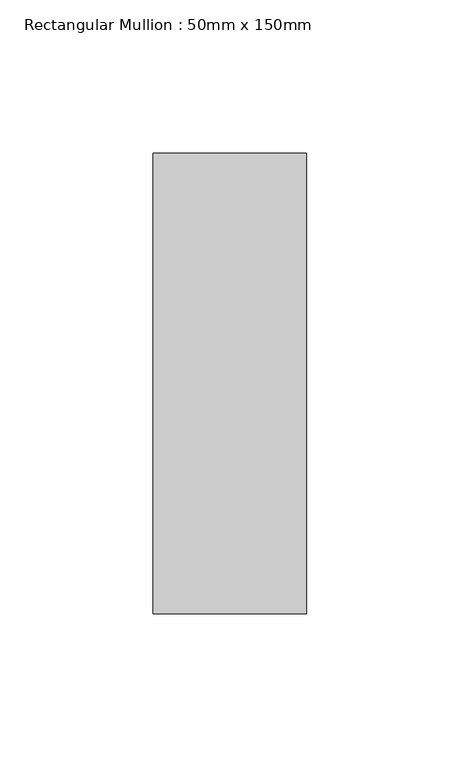
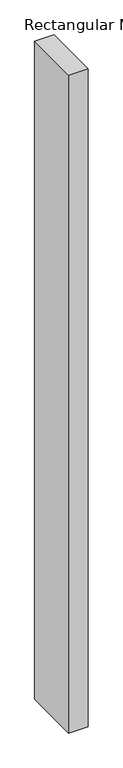
"""IFC4 building model written with IfcOpenShell, lengths in millimetres: member geometry, Rectangular Mullion : 50mm x 150mm."""

from ifc_helpers import new_model, si_unit, frame, origin, place, context, project, spatial, polyline, outline, extrude, source, transform, mapped, element, save


def rectangular_mullion_50mm_x_150mm_ded00a16(model_context):
    return source(origin(), model_context, "Body", "SweptSolid", [
        extrude(outline(polyline([(0.0, 75.0), (0.0, -75.0), (-50.0, -75.0), (-50.0, 75.0), (0.0, 75.0)])), frame((0.0, 0.0, -1780.0), z_axis=(0.0, 0.0, 1.0), x_axis=(1.0, 0.0, 0.0)), (0.0, 0.0, 1.0), 1780.0),
    ])


if __name__ == "__main__":
    model = new_model("IFC4")
    model_context = context("Model", 3, world=origin())
    ifc_project = project(units=[si_unit("LENGTHUNIT", "METRE", prefix="MILLI")], contexts=[model_context])
    site = spatial("IfcSite", under=ifc_project)
    building = spatial("IfcBuilding", under=site)
    placement = place(None, origin())
    rectangular_mullion_50mm_x_150mm_shape = rectangular_mullion_50mm_x_150mm_ded00a16(model_context)
    element("IfcMember", 1, ObjectType="Rectangular Mullion : 50mm x 150mm", at=placement, inside=building, context=model_context, shape_type="MappedRepresentation", body=[
        mapped(rectangular_mullion_50mm_x_150mm_shape, transform((0.0, 0.0, 0.0), x_axis=(1.0, 0.0, 0.0), y_axis=(0.0, 1.0, 0.0), z_axis=(0.0, 0.0, 1.0))),
    ])
    save(model, "model.ifc")

# Revit data of these elements
# Type "Rectangular Mullion : 50mm x 150mm"
#   built-in parameter 1007304 = 0.492126 (stored number, unit not read)
#   built-in parameter 1007301 = 0.082021 (stored number, unit not read)
#   built-in parameter 1007300 = 0.082021 (stored number, unit not read)
# Element 1 (IfcMember, "Rectangular Mullion : 50mm x 150mm")
#   Materials on its faces: "Aluminum"
# Materials
#   "Aluminum": class "Metal", colour RGB 244 244 244, transparency 0, Description = "Aluminum 6061", Cost = 0
